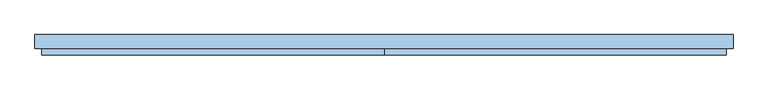
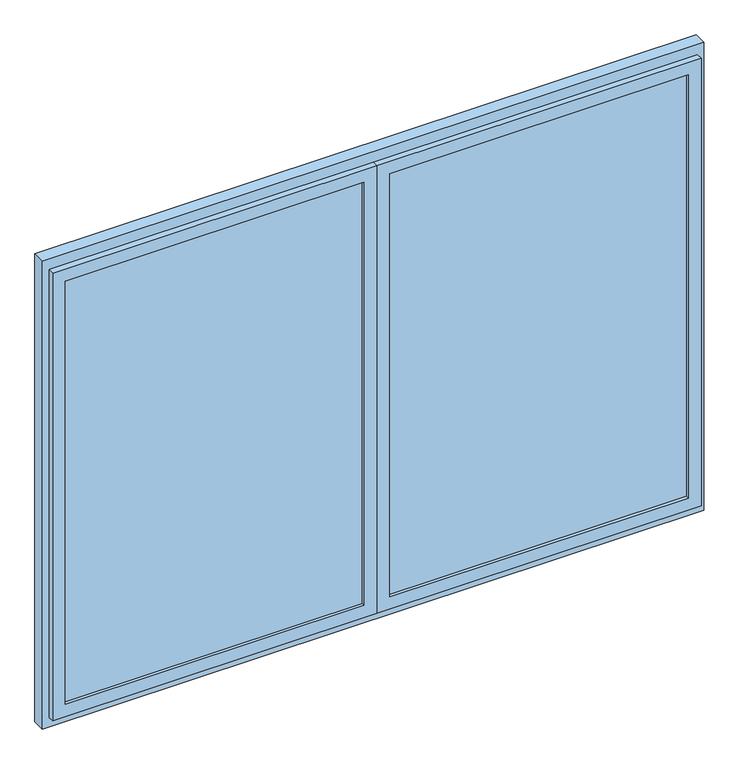
"""IFC4 building model written with IfcOpenShell, lengths in millimetres: window geometry, Fenstertür 2-flg : Fenstertür 2-flg 3.075x2.3."""

from ifc_helpers import new_model, si_unit, frame, origin, place, context, project, spatial, polyline, outline, extrude, faceted_brep, source, transform, mapped, element, save


def window_12bcd0c4(model_context):
    return source(origin(), model_context, "Body", "SolidModel", [
        extrude(outline(polyline([(30.0, -30.0), (-30.0, -30.0), (-30.0, 30.0), (30.0, 30.0), (30.0, -30.0)])), frame((0.0, 0.0, 80.0), z_axis=(0.0, 0.0, 1.0), x_axis=(1.0, 0.0, 0.0)), (0.0, 0.0, 1.0), 2140.0),
        extrude(outline(polyline([(2300.0, -1537.5), (0.0, -1537.5), (0.0, 1537.5), (2300.0, 1537.5), (2300.0, -1537.5)]), holes=[polyline([(2220.0, -1477.5), (2220.0, 1477.5), (80.0, 1477.5), (80.0, -1477.5), (2220.0, -1477.5)])]), frame((0.0, -30.0, 0.0), z_axis=(0.0, 1.0, 0.0), x_axis=(0.0, 0.0, 1.0)), (0.0, 0.0, 1.0), 60.0),
        faceted_brep([(-1477.5, -30.0, 80.0), (-1477.5, 0.0, 80.0), (-30.0, 0.0, 80.0), (-30.0, -30.0, 80.0), (-30.0, 0.0, 2220.0), (-30.0, -30.0, 2220.0), (-1477.5, 0.0, 2220.0), (-60.0, 0.0, 2190.0), (-1447.5, 0.0, 2190.0), (-1447.5, 0.0, 110.0), (-60.0, 0.0, 110.0), (0.0, -30.0, 50.0), (-1507.5, -30.0, 50.0), (-1507.5, -30.0, 2250.0), (0.0, -30.0, 2250.0), (-1477.5, -30.0, 2220.0), (-1507.5, -60.0, 50.0), (0.0, -60.0, 50.0), (0.0, -60.0, 2250.0), (-1507.5, -60.0, 2250.0), (-60.0, -60.0, 110.0), (-1447.5, -60.0, 110.0), (-1447.5, -60.0, 2190.0), (-60.0, -60.0, 2190.0)], [[[0, 1, 2, 3]], [[3, 2, 4, 5]], [[2, 1, 6, 4], [7, 8, 9, 10]], [[11, 12, 13, 14], [5, 15, 0, 3]], [[16, 12, 11, 17]], [[17, 11, 14, 18]], [[18, 19, 16, 17], [20, 21, 22, 23]], [[9, 21, 20, 10]], [[10, 20, 23, 7]], [[15, 6, 1, 0]], [[19, 13, 12, 16]], [[8, 22, 21, 9]], [[5, 4, 6, 15]], [[18, 14, 13, 19]], [[7, 23, 22, 8]]]),
        faceted_brep([(30.0, -30.0, 80.0), (30.0, 0.0, 80.0), (1477.5, 0.0, 80.0), (1477.5, -30.0, 80.0), (1477.5, 0.0, 2220.0), (1477.5, -30.0, 2220.0), (30.0, 0.0, 2220.0), (1447.5, 0.0, 2190.0), (60.0, 0.0, 2190.0), (60.0, 0.0, 110.0), (1447.5, 0.0, 110.0), (1507.5, -30.0, 50.0), (0.0, -30.0, 50.0), (0.0, -30.0, 2250.0), (1507.5, -30.0, 2250.0), (30.0, -30.0, 2220.0), (0.0, -60.0, 50.0), (1507.5, -60.0, 50.0), (1507.5, -60.0, 2250.0), (0.0, -60.0, 2250.0), (1447.5, -60.0, 110.0), (60.0, -60.0, 110.0), (60.0, -60.0, 2190.0), (1447.5, -60.0, 2190.0)], [[[0, 1, 2, 3]], [[3, 2, 4, 5]], [[2, 1, 6, 4], [7, 8, 9, 10]], [[11, 12, 13, 14], [5, 15, 0, 3]], [[16, 12, 11, 17]], [[17, 11, 14, 18]], [[18, 19, 16, 17], [20, 21, 22, 23]], [[9, 21, 20, 10]], [[10, 20, 23, 7]], [[15, 6, 1, 0]], [[19, 13, 12, 16]], [[8, 22, 21, 9]], [[5, 4, 6, 15]], [[18, 14, 13, 19]], [[7, 23, 22, 8]]]),
        extrude(outline(polyline([(60.0, -15.0), (1447.5, -15.0), (1447.5, -45.0), (60.0, -45.0), (60.0, -15.0)])), frame((0.0, 0.0, 110.0), z_axis=(0.0, 0.0, 1.0), x_axis=(1.0, 0.0, 0.0)), (0.0, 0.0, 1.0), 2080.0),
        extrude(outline(polyline([(-1447.5, -15.0), (-60.0, -15.0), (-60.0, -45.0), (-1447.5, -45.0), (-1447.5, -15.0)])), frame((0.0, 0.0, 110.0), z_axis=(0.0, 0.0, 1.0), x_axis=(1.0, 0.0, 0.0)), (0.0, 0.0, 1.0), 2080.0),
    ])


if __name__ == "__main__":
    model = new_model("IFC4")
    model_context = context("Model", 3, world=origin())
    ifc_project = project(units=[si_unit("LENGTHUNIT", "METRE", prefix="MILLI")], contexts=[model_context])
    site = spatial("IfcSite", under=ifc_project)
    building = spatial("IfcBuilding", under=site)
    placement = place(None, origin())
    window_shape = window_12bcd0c4(model_context)
    element("IfcWindow", 1, ObjectType="Fenstertür 2-flg : Fenstertür 2-flg 3.075x2.3", at=placement, inside=building, context=model_context, shape_type="MappedRepresentation", body=[
        mapped(window_shape, transform((0.0, 0.0, 0.0), x_axis=(1.0, 0.0, 0.0), y_axis=(0.0, 1.0, 0.0), z_axis=(0.0, 0.0, 1.0))),
    ])
    save(model, "model.ifc")

# Revit data of these elements
# Type "Fenstertür 2-flg : Fenstertür 2-flg 3.075x2.3"
#   Type Mark = "75"
#   Operation = "DoublePanelVertical"
#   Construction Type Id = "GSP4R"
#   Keynote = "16.05.01"
#   Analytic Construction = "1/8 Zoll Pilkington-Verglasung einfach"
#   Thermal Resistance (R) = 0.271106 (m²·K)/W
#   Visual Light Transmittance = 0.9
#   Solar Heat Gain Coefficient = 0.78
#   Rough Width = 3.075 m
#   Rough Height = 2.300 m
#   Heat Transfer Coefficient (U) = 3.6886 W/(m²·K)
#   Rahmentiefe = 0.060 m
#   Rahmenhöhe unten = 0.080 m
#   Höhe oberer  Rahmen = 0.080 m
#   Rahmenbreite = 0.060 m
#   Height = 2.300 m
#   Tiefe Flügel = 0.060 m
#   Flügelbreite = 0.060 m
#   Einbautiefe (von außen) [instance default] = 0.140 m
#   Width = 3.075 m
#   Sichtbarkeit Sturzlinien [instance default] = yes
#   Öffnungsrichtung oben [instance default] = yes
#   Öffnungsrichtung in Draufsicht anzeigen [instance default] = yes
#   Drehflügel 1 [instance default] = yes
#   Bild [instance default] = none
#   Glas [instance default] = none
#   Fensterflügel [instance default] = none
#   Äußere Fensterbank [instance default] = none
#   Innere Fensterbank [instance default] = none
#   Wall Closure = (empty or 0)
# Element 1 (IfcWindow, "Fenstertür 2-flg : Fenstertür 2-flg 3.075x2.3")
#   Einbautiefe (von außen) = 0.120 m
#   Materials on its faces: "Kunststoff - Weiß", "Glas"
# Materials
#   "Kunststoff - Weiß": class "Kunststoff", colour RGB 249 249 249, transparency 0, Cost = 0
#   "Glas": class "Glas", colour RGB 0 0 255, transparency 0.75, Comments = "Render-Darstellung nicht aktualisiert ", Cost = 0
